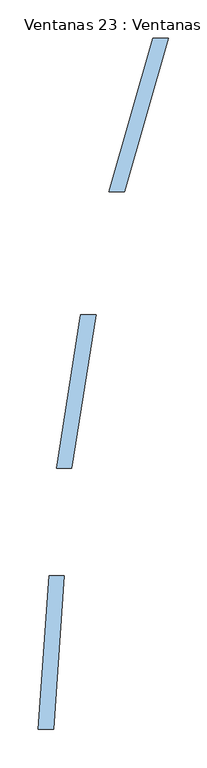
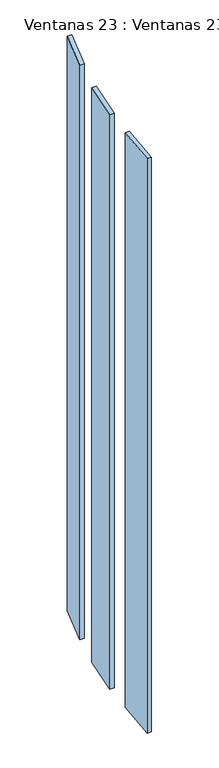
"""IFC4 building model written with IfcOpenShell, lengths in millimetres: window geometry, Ventanas 23 : Ventanas 23."""

from ifc_helpers import new_model, si_unit, frame, origin, place, context, project, spatial, polyline, outline, extrude, source, transform, mapped, element, save


def ventanas_23_ventanas_23_febadd23(model_context):
    return source(origin(), model_context, "Body", "SweptSolid", [
        extrude(outline(polyline([(-1476.1519788, 3714.5805588), (-1456.1519788, 3714.5805588), (-1470.1373412, 3514.5805588), (-1490.1373412, 3514.5805588), (-1476.1519788, 3714.5805588)])), frame((0.0, 0.0, 6100.0), z_axis=(0.0, 0.0, 1.0), x_axis=(1.0, 0.0, 0.0)), (0.0, 0.0, 1.0), 2815.3215694),
        extrude(outline(polyline([(-1434.685337, 4054.5805588), (-1414.685337, 4054.5805588), (-1446.3622251, 3854.5805588), (-1466.3622251, 3854.5805588), (-1434.685337, 4054.5805588)])), frame((0.0, 0.0, 6100.0), z_axis=(0.0, 0.0, 1.0), x_axis=(1.0, 0.0, 0.0)), (0.0, 0.0, 1.0), 2815.3215694),
        extrude(outline(polyline([(-1340.3973493, 4414.5805588), (-1320.3973493, 4414.5805588), (-1377.7464265, 4214.5805588), (-1397.7464265, 4214.5805588), (-1340.3973493, 4414.5805588)])), frame((0.0, 0.0, 6100.0), z_axis=(0.0, 0.0, 1.0), x_axis=(1.0, 0.0, 0.0)), (0.0, 0.0, 1.0), 2815.3215694),
    ])


if __name__ == "__main__":
    model = new_model("IFC4")
    model_context = context("Model", 3, world=origin())
    ifc_project = project(units=[si_unit("LENGTHUNIT", "METRE", prefix="MILLI")], contexts=[model_context])
    site = spatial("IfcSite", under=ifc_project)
    building = spatial("IfcBuilding", under=site)
    placement = place(None, origin())
    ventanas_23_ventanas_23_shape = ventanas_23_ventanas_23_febadd23(model_context)
    element("IfcWindow", 1, ObjectType="Ventanas 23 : Ventanas 23", at=placement, inside=building, context=model_context, shape_type="MappedRepresentation", body=[
        mapped(ventanas_23_ventanas_23_shape, transform((0.0, 0.0, 0.0), x_axis=(1.0, 0.0, 0.0), y_axis=(0.0, 1.0, 0.0), z_axis=(0.0, 0.0, 1.0))),
    ])
    save(model, "model.ifc")

# Revit data of these elements
# Type "Ventanas 23 : Ventanas 23"
#   Type Mark = "51"
# Element 1 (IfcWindow, "Ventanas 23 : Ventanas 23")
#   Materials on its faces: "VIDRIO"
# Materials
#   "VIDRIO": class "Genérico", colour RGB 120 120 120, transparency 0, Cost = 0
